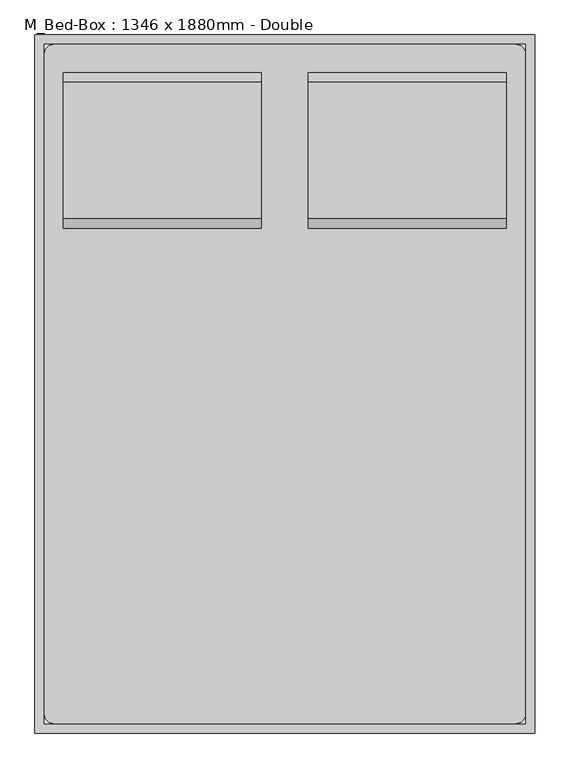
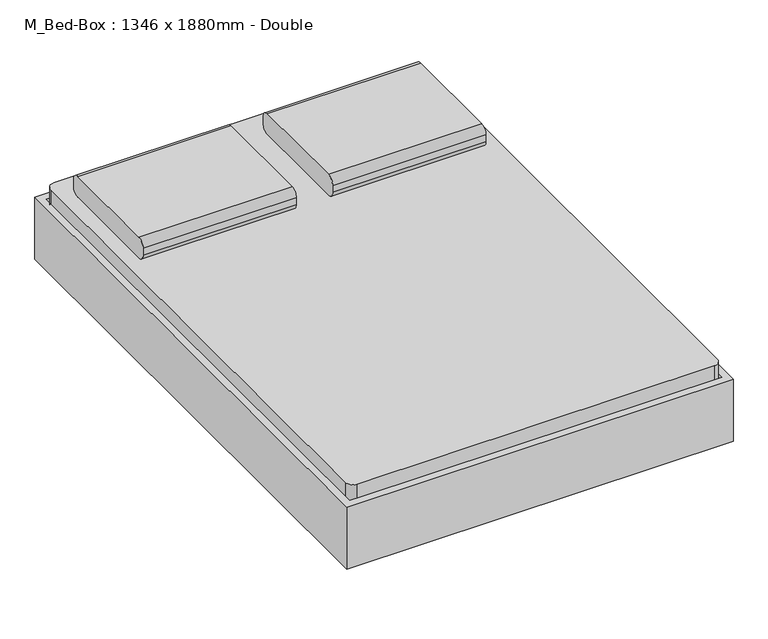
"""IFC4 building model written with IfcOpenShell, lengths in millimetres: furniture geometry, M_Bed-Box : 1346 x 1880mm - Double."""

import ifcopenshell
import ifcopenshell.guid

model = None  # the IFC model being written
_history = None  # IfcOwnerHistory: only IFC2X3 demands one
_inside = {}  # id of a spatial element -> (the spatial element, [elements in it])
_under = {}  # id of a project, library or spatial element -> (it, [spatial elements below it])
_declared = {}  # id of a project -> (the project, [libraries it declares])
_typed = {}  # id of a type object -> (the type object, [elements of that type])
_made_of = {}  # id of a material, layer set ... -> (it, [elements and type objects made of it])


def new_model(schema):
    """Start an empty IFC model of exactly this schema.

    Asked for "IFC4X3", IfcOpenShell would pick the latest addendum, in which some entities
    have other attributes; the version numbers below select the first issue.
    IFC2X3 requires an IfcOwnerHistory on every rooted entity: one is made here for all.
    """
    global model, _history
    if schema == "IFC4X3":
        model = ifcopenshell.file(schema_version=(4, 3, 0, 0))
    else:
        model = ifcopenshell.file(schema=schema)
    _inside.clear()
    _under.clear()
    _declared.clear()
    _typed.clear()
    _made_of.clear()
    _history = None
    if model.schema == "IFC2X3":
        org = make("IfcOrganization", Name="unknown")
        user = make(
            "IfcPersonAndOrganization",
            ThePerson=make("IfcPerson", FamilyName="unknown"),
            TheOrganization=org,
        )
        app = make(
            "IfcApplication",
            ApplicationDeveloper=org,
            Version="unknown",
            ApplicationFullName="unknown",
            ApplicationIdentifier="unknown",
        )
        _history = make(
            "IfcOwnerHistory",
            OwningUser=user,
            OwningApplication=app,
            ChangeAction="ADDED",
            CreationDate=0,
        )
    return model


def make(cls, **values):
    """One entity of the class cls with the attributes given. An attribute that is None is left unset."""
    return model.create_entity(
        cls, **{name: value for name, value in values.items() if value is not None}
    )


def rooted(cls, **values):
    """An entity with a GlobalId (a new one), such as an element, a storey or a relation."""
    return make(cls, GlobalId=ifcopenshell.guid.new(), OwnerHistory=_history, **values)


def si_unit(unit_type, name, prefix=None):
    """IfcSIUnit, for example si_unit("LENGTHUNIT", "METRE", prefix="MILLI")."""
    return make("IfcSIUnit", UnitType=unit_type, Prefix=prefix, Name=name)


def assignment(units):
    """IfcUnitAssignment: the units of a project."""
    return None if units is None else make("IfcUnitAssignment", Units=units)


def point(xyz):
    """IfcCartesianPoint."""
    return None if xyz is None else make("IfcCartesianPoint", Coordinates=xyz)


def direction(xyz):
    """IfcDirection."""
    return None if xyz is None else make("IfcDirection", DirectionRatios=xyz)


def frame(location, z_axis=None, x_axis=None):
    """IfcAxis2Placement3D, a coordinate frame: its origin and axes. An axis left out is left unset."""
    return make(
        "IfcAxis2Placement3D",
        Location=point(location),
        Axis=direction(z_axis),
        RefDirection=direction(x_axis),
    )


def frame_2d(location, x_axis=None):
    """IfcAxis2Placement2D, a coordinate frame in the plane: its origin and x axis."""
    return make(
        "IfcAxis2Placement2D", Location=point(location), RefDirection=direction(x_axis)
    )


def origin():
    """The frame at (0, 0, 0) with its axes left unset."""
    return frame((0.0, 0.0, 0.0))


def place(relative_to, where):
    """IfcLocalPlacement: puts the frame where relative to a parent placement (None: the world)."""
    return make(
        "IfcLocalPlacement", PlacementRelTo=relative_to, RelativePlacement=where
    )


def context(
    kind, dimensions, precision=None, world=None, true_north=None, identifier=None
):
    """IfcGeometricRepresentationContext, for example the 3D "Model" context."""
    return make(
        "IfcGeometricRepresentationContext",
        ContextIdentifier=identifier,
        ContextType=kind,
        CoordinateSpaceDimension=dimensions,
        Precision=precision,
        WorldCoordinateSystem=world,
        TrueNorth=true_north,
    )


def project(units=None, contexts=None):
    """IfcProject with its units and contexts."""
    return rooted(
        "IfcProject",
        Name="project",
        RepresentationContexts=contexts,
        UnitsInContext=assignment(units),
    )


def spatial(cls, under=None, at=None, **own):
    """A site, building, storey or space (cls), placed at a placement, below another one or the project."""
    s = rooted(cls, ObjectPlacement=at, **own)
    if under is not None:
        _under.setdefault(under.id(), (under, []))[1].append(s)
    return s


def polyline(points):
    """IfcPolyline through the points."""
    return make("IfcPolyline", Points=[point(p) for p in points])


def circle_curve(where, radius):
    """IfcCircle in the frame where."""
    return make("IfcCircle", Position=where, Radius=radius)


def trimmed(basis, trim1, trim2, sense, master):
    """IfcTrimmedCurve: the piece of a basis curve between two trims."""
    return make(
        "IfcTrimmedCurve",
        BasisCurve=basis,
        Trim1=trim1,
        Trim2=trim2,
        SenseAgreement=sense,
        MasterRepresentation=master,
    )


def segment(curve, same_sense, transition):
    """IfcCompositeCurveSegment."""
    return make(
        "IfcCompositeCurveSegment",
        Transition=transition,
        SameSense=same_sense,
        ParentCurve=curve,
    )


def composite_curve(segments, self_intersect=None):
    """IfcCompositeCurve: segments joined end to end."""
    return make("IfcCompositeCurve", Segments=segments, SelfIntersect=self_intersect)


def outline(outer, holes=None, kind="AREA"):
    """IfcArbitraryClosedProfileDef: a profile drawn as a closed curve; with holes, ...WithVoids."""
    if holes is None:
        return make("IfcArbitraryClosedProfileDef", ProfileType=kind, OuterCurve=outer)
    return make(
        "IfcArbitraryProfileDefWithVoids",
        ProfileType=kind,
        OuterCurve=outer,
        InnerCurves=holes,
    )


def extrude(swept, where, along, depth):
    """IfcExtrudedAreaSolid: the profile swept, set in the frame where, extruded along a direction by depth."""
    return make(
        "IfcExtrudedAreaSolid",
        SweptArea=swept,
        Position=where,
        ExtrudedDirection=direction(along),
        Depth=depth,
    )


def shape(context_of_items, identifier, shape_type, items):
    """IfcShapeRepresentation: the items that make up one representation, for example the "Body"."""
    return make(
        "IfcShapeRepresentation",
        ContextOfItems=context_of_items,
        RepresentationIdentifier=identifier,
        RepresentationType=shape_type,
        Items=items,
    )


def source(mapping_origin, context_of_items, identifier, shape_type, items):
    """IfcRepresentationMap: a shape defined once, which mapped items show again and again."""
    return make(
        "IfcRepresentationMap",
        MappingOrigin=mapping_origin,
        MappedRepresentation=shape(context_of_items, identifier, shape_type, items),
    )


def transform(
    local_origin,
    x_axis=None,
    y_axis=None,
    z_axis=None,
    scale=None,
    scale2=None,
    scale3=None,
    uniform=True,
):
    """IfcCartesianTransformationOperator3D, or its non-uniform kind. x_axis, y_axis, z_axis: its Axis1, 2, 3."""
    if uniform:
        return make(
            "IfcCartesianTransformationOperator3D",
            Axis1=direction(x_axis),
            Axis2=direction(y_axis),
            LocalOrigin=point(local_origin),
            Scale=scale,
            Axis3=direction(z_axis),
        )
    return make(
        "IfcCartesianTransformationOperator3DnonUniform",
        Axis1=direction(x_axis),
        Axis2=direction(y_axis),
        LocalOrigin=point(local_origin),
        Scale=scale,
        Axis3=direction(z_axis),
        Scale2=scale2,
        Scale3=scale3,
    )


def mapped(mapping_source, mapping_target):
    """IfcMappedItem: shows the shape of a source again, moved by a transform."""
    return make(
        "IfcMappedItem", MappingSource=mapping_source, MappingTarget=mapping_target
    )


def made_of(thing, what):
    """Note that an element or type object is made of a material, layer set ...; save() writes the relation."""
    if what is not None:
        _made_of.setdefault(what.id(), (what, []))[1].append(thing)
    return thing


def element(
    cls,
    number,
    at=None,
    inside=None,
    cuts=None,
    type_object=None,
    material=None,
    context=None,
    identifier="Body",
    shape_type=None,
    held_by="IfcProductDefinitionShape",
    body=None,
    shapes=None,
    **own,
):
    """One element of the class cls, such as IfcWall. Its Tag is "e" and its number.

    at: its placement. inside: the storey or other place that contains it. cuts: it is an
    opening in that element (IfcRelVoidsElement). A single representation is given by context,
    identifier, shape_type and body (its items); several are given by shapes. held_by: the class
    of the entity that holds the representations. save() writes the other relations.
    """
    e = rooted(cls, Tag="e%d" % number, ObjectPlacement=at, **own)
    if body is not None:
        shapes = [shape(context, identifier, shape_type, body)]
    if shapes is not None:
        e.Representation = make(held_by, Representations=shapes)
    if inside is not None:
        _inside.setdefault(inside.id(), (inside, []))[1].append(e)
    if cuts is not None:
        rooted(
            "IfcRelVoidsElement", RelatingBuildingElement=cuts, RelatedOpeningElement=e
        )
    if type_object is not None:
        _typed.setdefault(type_object.id(), (type_object, []))[1].append(e)
    return made_of(e, material)


def aggregate(whole, parts):
    """IfcRelAggregates: a whole, such as a stair, and the parts it consists of."""
    return rooted("IfcRelAggregates", RelatingObject=whole, RelatedObjects=parts)


def save(model, path):
    """Write the relations noted so far, then the file.

    IfcRelAggregates (storeys below a building ...), IfcRelContainedInSpatialStructure (elements
    in a storey), IfcRelDefinesByType, IfcRelAssociatesMaterial and IfcRelDeclares: one each for
    every whole, place, type object, material and project.
    """
    for whole, parts in _under.values():
        aggregate(whole, parts)
    for where, things in _inside.values():
        rooted(
            "IfcRelContainedInSpatialStructure",
            RelatedElements=things,
            RelatingStructure=where,
        )
    for kind, things in _typed.values():
        rooted("IfcRelDefinesByType", RelatedObjects=things, RelatingType=kind)
    for what, things in _made_of.values():
        rooted("IfcRelAssociatesMaterial", RelatedObjects=things, RelatingMaterial=what)
    for by, libraries in _declared.values():
        rooted("IfcRelDeclares", RelatingContext=by, RelatedDefinitions=libraries)
    model.write(path)


def plane_surface(at):
    """IfcPlane: the flat surface through the origin of the frame at, square to its z axis."""
    return make("IfcPlane", Position=at)


def cylinder_surface(at, radius):
    """IfcCylindricalSurface: all points at the distance radius from the z axis of the frame at."""
    return make("IfcCylindricalSurface", Position=at, Radius=radius)


def revolved_surface(curve, axis_point, axis_direction):
    """IfcSurfaceOfRevolution: the curve turned about the line through axis_point along axis_direction."""
    return make(
        "IfcSurfaceOfRevolution",
        SweptCurve=make("IfcArbitraryOpenProfileDef", ProfileType="CURVE", Curve=curve),
        AxisPosition=make("IfcAxis1Placement", Location=point(axis_point), Axis=direction(axis_direction)),
    )


def advanced_brep(points, edges, surfaces, faces):
    """IfcAdvancedBrep: a solid bounded by faces that lie on surfaces and meet in shared edges.

    An edge is (start, end): straight between two places in points (the first is 0);
    or (start, end, curve); or (start, end, curve, False) where it runs against its curve.
    A face is (place in surfaces, loops), or (place, loops, False) where it looks against
    its surface's normal. A loop lists edges by number (the first is 1), with a minus sign
    where the edge is run from its end to its start. The first loop is the outer one.
    """
    corners = [point(p) for p in points]
    vertices = [make("IfcVertexPoint", VertexGeometry=c) for c in corners]
    made = []
    for start, end, *more in edges:
        made.append(
            make(
                "IfcEdgeCurve",
                EdgeStart=vertices[start],
                EdgeEnd=vertices[end],
                EdgeGeometry=more[0] if more else make("IfcPolyline", Points=[corners[start], corners[end]]),
                SameSense=more[1] if len(more) > 1 else True,
            )
        )
    hull = []
    for where, loops, *sense in faces:
        bounds = []
        for j, loop in enumerate(loops):
            ring = [make("IfcOrientedEdge", EdgeElement=made[abs(k) - 1], Orientation=k > 0) for k in loop]
            bounds.append(
                make(
                    "IfcFaceOuterBound" if j == 0 else "IfcFaceBound",
                    Bound=make("IfcEdgeLoop", EdgeList=ring),
                    Orientation=True,
                )
            )
        hull.append(make("IfcAdvancedFace", Bounds=bounds, FaceSurface=surfaces[where], SameSense=sense[0] if sense else True))
    return make("IfcAdvancedBrep", Outer=make("IfcClosedShell", CfsFaces=hull))


def m_bed_box_1346_x_1880mm_double_b32eb57e(model_context):
    return source(origin(), model_context, "Body", "SolidModel", [
        extrude(outline(composite_curve([segment(polyline([(578.5704918, 406.4), (210.2704918, 406.4)]), True, "CONTINUOUS"), segment(trimmed(circle_curve(frame_2d((210.2704918, 431.8)), 25.4), [point((210.2704918, 406.4))], [point((184.8704918, 431.8))], False, "CARTESIAN"), True, "CONTINUOUS"), segment(polyline([(184.8704918, 431.8), (184.8704918, 457.2)]), True, "CONTINUOUS"), segment(trimmed(circle_curve(frame_2d((210.2704918, 457.2)), 25.4), [point((184.8704918, 457.2))], [point((210.2704918, 482.6))], False, "CARTESIAN"), True, "CONTINUOUS"), segment(polyline([(210.2704918, 482.6), (578.5704918, 482.6)]), True, "CONTINUOUS"), segment(trimmed(circle_curve(frame_2d((578.5704918, 457.2)), 25.4), [point((578.5704918, 482.6))], [point((603.9704918, 457.2))], False, "CARTESIAN"), True, "CONTINUOUS"), segment(polyline([(603.9704918, 457.2), (603.9704918, 431.8)]), True, "CONTINUOUS"), segment(trimmed(circle_curve(frame_2d((578.5704918, 431.8)), 25.4), [point((603.9704918, 431.8))], [point((578.5704918, 406.4))], False, "CARTESIAN"), True, "CONTINUOUS")], self_intersect=False)), frame((402.652459, 0.0, 0.0), z_axis=(1.0, 0.0, 0.0), x_axis=(0.0, 1.0, 0.0)), (0.0, 0.0, 1.0), 533.3),
        extrude(outline(composite_curve([segment(polyline([(578.5704918, 406.4), (210.2704918, 406.4)]), True, "CONTINUOUS"), segment(trimmed(circle_curve(frame_2d((210.2704918, 431.8)), 25.4), [point((210.2704918, 406.4))], [point((184.8704918, 431.8))], False, "CARTESIAN"), True, "CONTINUOUS"), segment(polyline([(184.8704918, 431.8), (184.8704918, 457.2)]), True, "CONTINUOUS"), segment(trimmed(circle_curve(frame_2d((210.2704918, 457.2)), 25.4), [point((184.8704918, 457.2))], [point((210.2704918, 482.6))], False, "CARTESIAN"), True, "CONTINUOUS"), segment(polyline([(210.2704918, 482.6), (578.5704918, 482.6)]), True, "CONTINUOUS"), segment(trimmed(circle_curve(frame_2d((578.5704918, 457.2)), 25.4), [point((578.5704918, 482.6))], [point((603.9704918, 457.2))], False, "CARTESIAN"), True, "CONTINUOUS"), segment(polyline([(603.9704918, 457.2), (603.9704918, 431.8)]), True, "CONTINUOUS"), segment(trimmed(circle_curve(frame_2d((578.5704918, 431.8)), 25.4), [point((603.9704918, 431.8))], [point((578.5704918, 406.4))], False, "CARTESIAN"), True, "CONTINUOUS")], self_intersect=False)), frame((-257.647541, 0.0, 0.0), z_axis=(1.0, 0.0, 0.0), x_axis=(0.0, 1.0, 0.0)), (0.0, 0.0, 1.0), 533.3),
        advanced_brep(
        [(-308.1231784, 451.5704918, 177.8), (-308.1231784, 375.3704918, 177.8), (-308.1231784, 375.3704918, 196.85), (-308.1231784, 451.5704918, 196.85), (-257.3231784, 451.5704918, 177.8), (-257.3231784, 375.3704918, 177.8), (-245.1869899, 375.3704918, 196.85), (-245.1869899, 451.5704918, 196.85), (-181.2523099, 451.5704918, 14.6654962), (-181.2523099, 375.3704918, 14.6654962), (-163.9871466, 375.3704918, 22.716374), (-163.9871466, 451.5704918, 22.716374), (-158.2320921, 375.3704918, 0.0), (-158.2320921, 451.5704918, 0.0), (-158.2320921, 375.3704918, 19.05), (-158.2320921, 451.5704918, 19.05), (-79.6195862, 451.5704918, 0.0), (-79.6195862, 375.3704918, 0.0), (-79.6195862, 375.3704918, 19.05), (-79.6195862, 451.5704918, 19.05), (-66.9195862, 375.3704918, 3.4029547), (-66.9195862, 451.5704918, 3.4029547), (-76.4445862, 375.3704918, 19.9007387), (-76.4445862, 451.5704918, 19.9007387), (-6.822541, 451.5704918, 38.1), (-6.822541, 375.3704918, 38.1), (-11.9269731, 375.3704918, 57.15), (-11.9269731, 451.5704918, 57.15), (685.4518216, 451.5704918, 38.1), (685.4518216, 375.3704918, 38.1), (690.5562537, 375.3704918, 57.15), (690.5562537, 451.5704918, 57.15), (745.5488669, 451.5704918, 3.4029547), (745.5488669, 375.3704918, 3.4029547), (755.0738669, 375.3704918, 19.9007387), (755.0738669, 451.5704918, 19.9007387), (758.2488669, 375.3704918, 0.0), (758.2488669, 451.5704918, 0.0), (758.2488669, 375.3704918, 19.05), (758.2488669, 451.5704918, 19.05), (836.8613728, 451.5704918, 0.0), (836.8613728, 375.3704918, 0.0), (836.8613728, 375.3704918, 19.05), (836.8613728, 451.5704918, 19.05), (859.8815906, 375.3704918, 14.6654962), (859.8815906, 451.5704918, 14.6654962), (842.6164272, 375.3704918, 22.716374), (842.6164272, 451.5704918, 22.716374), (935.952459, 451.5704918, 177.8), (935.952459, 375.3704918, 177.8), (923.8162705, 375.3704918, 196.85), (923.8162705, 451.5704918, 196.85), (986.752459, 451.5704918, 177.8), (986.752459, 451.5704918, 196.85), (986.752459, 375.3704918, 196.85), (986.752459, 375.3704918, 177.8)],
        [
            (0, 1),
            (1, 2),
            (2, 3),
            (3, 0),
            (0, 4),
            (4, 5),
            (5, 1),
            (5, 6),
            (6, 2),
            (6, 7),
            (7, 3),
            (7, 4),
            (4, 8),
            (8, 9),
            (9, 5),
            (9, 10),
            (10, 6),
            (10, 11),
            (11, 7),
            (11, 8),
            (12, 9, circle_curve(frame((-158.2320921, 375.3704918, 25.4), z_axis=(0.0, 1.0, 0.0), x_axis=(-0.906307787036649, 0.0, -0.4226182617407015)), 25.4)),
            (8, 13, circle_curve(frame((-158.2320921, 451.5704918, 25.4), z_axis=(0.0, -1.0, 0.0), x_axis=(-0.906307787036649, 0.0, -0.4226182617407015)), 25.4)),
            (13, 12),
            (14, 10, circle_curve(frame((-158.2320921, 375.3704918, 25.4), z_axis=(0.0, 1.0, 0.0), x_axis=(-0.906307787036649, 0.0, -0.4226182617407015)), 6.35)),
            (12, 14),
            (15, 11, circle_curve(frame((-158.2320921, 451.5704918, 25.4), z_axis=(0.0, 1.0, 0.0), x_axis=(-0.906307787036649, 0.0, -0.4226182617407015)), 6.35)),
            (14, 15),
            (15, 13),
            (13, 16),
            (16, 17),
            (17, 12),
            (17, 18),
            (18, 14),
            (18, 19),
            (19, 15),
            (19, 16),
            (20, 17, circle_curve(frame((-79.6195862, 375.3704918, 25.4), z_axis=(0.0, 1.0, 0.0), x_axis=(0.0, 0.0, -1.0)), 25.4)),
            (16, 21, circle_curve(frame((-79.6195862, 451.5704918, 25.4), z_axis=(0.0, -1.0, 0.0), x_axis=(0.0, 0.0, -1.0)), 25.4)),
            (21, 20),
            (22, 18, circle_curve(frame((-79.6195862, 375.3704918, 25.4), z_axis=(0.0, 1.0, 0.0), x_axis=(0.0, 0.0, -1.0)), 6.35)),
            (20, 22),
            (23, 19, circle_curve(frame((-79.6195862, 451.5704918, 25.4), z_axis=(0.0, 1.0, 0.0), x_axis=(0.0, 0.0, -1.0)), 6.35)),
            (22, 23),
            (23, 21),
            (21, 24),
            (24, 25),
            (25, 20),
            (25, 26),
            (26, 22),
            (26, 27),
            (27, 23),
            (27, 24),
            (24, 28),
            (28, 29),
            (29, 25),
            (29, 30),
            (30, 26),
            (30, 31),
            (31, 27),
            (31, 28),
            (28, 32),
            (32, 33),
            (33, 29),
            (33, 34),
            (34, 30),
            (34, 35),
            (35, 31),
            (35, 32),
            (36, 33, circle_curve(frame((758.2488669, 375.3704918, 25.4), z_axis=(0.0, 1.0, 0.0), x_axis=(-0.5000000000000463, 0.0, -0.8660254037844118)), 25.4)),
            (32, 37, circle_curve(frame((758.2488669, 451.5704918, 25.4), z_axis=(0.0, -1.0, 0.0), x_axis=(-0.5000000000000463, 0.0, -0.8660254037844118)), 25.4)),
            (37, 36),
            (38, 34, circle_curve(frame((758.2488669, 375.3704918, 25.4), z_axis=(0.0, 1.0, 0.0), x_axis=(-0.5000000000000463, 0.0, -0.8660254037844118)), 6.35)),
            (36, 38),
            (39, 35, circle_curve(frame((758.2488669, 451.5704918, 25.4), z_axis=(0.0, 1.0, 0.0), x_axis=(-0.5000000000000463, 0.0, -0.8660254037844118)), 6.35)),
            (38, 39),
            (39, 37),
            (37, 40),
            (40, 41),
            (41, 36),
            (41, 42),
            (42, 38),
            (42, 43),
            (43, 39),
            (43, 40),
            (44, 41, circle_curve(frame((836.8613728, 375.3704918, 25.4), z_axis=(0.0, 1.0, 0.0), x_axis=(0.0, 0.0, -1.0)), 25.4)),
            (40, 45, circle_curve(frame((836.8613728, 451.5704918, 25.4), z_axis=(0.0, -1.0, 0.0), x_axis=(0.0, 0.0, -1.0)), 25.4)),
            (45, 44),
            (46, 42, circle_curve(frame((836.8613728, 375.3704918, 25.4), z_axis=(0.0, 1.0, 0.0), x_axis=(0.0, 0.0, -1.0)), 6.35)),
            (44, 46),
            (47, 43, circle_curve(frame((836.8613728, 451.5704918, 25.4), z_axis=(0.0, 1.0, 0.0), x_axis=(0.0, 0.0, -1.0)), 6.35)),
            (46, 47),
            (47, 45),
            (45, 48),
            (48, 49),
            (49, 44),
            (49, 50),
            (50, 46),
            (50, 51),
            (51, 47),
            (51, 48),
            (52, 53),
            (53, 54),
            (54, 55),
            (55, 52),
            (48, 52),
            (55, 49),
            (54, 50),
            (53, 51),
        ],
        [
            plane_surface(frame((-308.1231784, 705.5704918, -152.9490627), z_axis=(-1.0, 0.0, 0.0), x_axis=(0.0, 1.0, 0.0))),
            plane_surface(frame((-308.1231784, 451.5704918, 177.8), z_axis=(0.0, 0.0, -1.0), x_axis=(1.0, 0.0, 0.0))),
            plane_surface(frame((-308.1231784, 375.3704918, 177.8), z_axis=(0.0, -1.0, 0.0), x_axis=(1.0, 0.0, 0.0))),
            plane_surface(frame((-308.1231784, 375.3704918, 196.85), z_axis=(0.0, 0.0, 1.0), x_axis=(1.0, 0.0, 0.0))),
            plane_surface(frame((-308.1231784, 451.5704918, 196.85), z_axis=(0.0, 1.0, 0.0), x_axis=(1.0, 0.0, 0.0))),
            plane_surface(frame((-257.3231784, 451.5704918, 177.8), z_axis=(-0.9063077870366486, 0.0, -0.4226182617407026), x_axis=(0.4226182617407026, 0.0, -0.9063077870366486))),
            plane_surface(frame((-257.3231784, 375.3704918, 177.8), z_axis=(0.0, -1.0000000000000002, 0.0), x_axis=(0.4226182617407026, 0.0, -0.9063077870366486))),
            plane_surface(frame((-245.1869899, 375.3704918, 196.85), z_axis=(0.9063077870366487, 0.0, 0.4226182617407023), x_axis=(0.4226182617407023, 0.0, -0.9063077870366487))),
            plane_surface(frame((-245.1869899, 451.5704918, 196.85), z_axis=(0.0, 1.0, 0.0), x_axis=(0.4226182617407027, 0.0, -0.9063077870366485))),
            cylinder_surface(frame((-158.2320921, 705.5704918, 25.4), z_axis=(0.0, -1.0, 0.0), x_axis=(-0.906307787036649, 0.0, -0.4226182617407015)), 25.4),
            plane_surface(frame((-158.2320921, 375.3704918, 25.4), z_axis=(0.0, -1.0, 0.0), x_axis=(-0.906307787036649, 0.0, -0.4226182617407015))),
            revolved_surface(polyline([(-163.9871465476827, 375.3704918, 22.716374037946544), (-163.9871465476827, 451.5704918, 22.716374037946544)]), (-158.2320921, 705.5704918, 25.4), (0.0, -1.0, 0.0)),
            plane_surface(frame((-158.2320921, 451.5704918, 25.4), z_axis=(0.0, 1.0, 0.0), x_axis=(-0.906307787036649, 0.0, -0.4226182617407015))),
            plane_surface(frame((-158.2320921, 451.5704918, 0.0), z_axis=(0.0, 0.0, -1.0), x_axis=(1.0, 0.0, 0.0))),
            plane_surface(frame((-158.2320921, 375.3704918, 0.0), z_axis=(0.0, -1.0, 0.0), x_axis=(1.0, 0.0, 0.0))),
            plane_surface(frame((-158.2320921, 375.3704918, 19.05), z_axis=(0.0, 0.0, 1.0), x_axis=(1.0, 0.0, 0.0))),
            plane_surface(frame((-158.2320921, 451.5704918, 19.05), z_axis=(0.0, 1.0, 0.0), x_axis=(1.0, 0.0, 0.0))),
            cylinder_surface(frame((-79.6195862, 705.5704918, 25.4), z_axis=(0.0, -1.0, 0.0), x_axis=(0.0, 0.0, -1.0)), 25.4),
            plane_surface(frame((-79.6195862, 375.3704918, 25.4), z_axis=(0.0, -1.0, 0.0), x_axis=(0.0, 0.0, -1.0))),
            revolved_surface(polyline([(-79.6195862, 375.3704918, 19.049999999999997), (-79.6195862, 451.5704918, 19.049999999999997)]), (-79.6195862, 705.5704918, 25.4), (0.0, -1.0, 0.0)),
            plane_surface(frame((-79.6195862, 451.5704918, 25.4), z_axis=(0.0, 1.0, 0.0), x_axis=(0.0, 0.0, -1.0))),
            plane_surface(frame((-66.9195862, 451.5704918, 3.4029547), z_axis=(0.4999999999998744, 0.0, -0.8660254037845112), x_axis=(0.8660254037845112, 0.0, 0.4999999999998744))),
            plane_surface(frame((-66.9195862, 375.3704918, 3.4029547), z_axis=(0.0, -1.0000000000000002, 0.0), x_axis=(0.8660254037845112, 0.0, 0.4999999999998745))),
            plane_surface(frame((-76.4445862, 375.3704918, 19.9007387), z_axis=(-0.4999999999998741, 0.0, 0.8660254037845113), x_axis=(0.8660254037845113, 0.0, 0.4999999999998741))),
            plane_surface(frame((-76.4445862, 451.5704918, 19.9007387), z_axis=(0.0, 1.0, 0.0), x_axis=(0.866025403784511, 0.0, 0.49999999999987477))),
            plane_surface(frame((-6.822541, 451.5704918, 38.1), z_axis=(0.0, 0.0, -1.0), x_axis=(1.0, 0.0, 0.0))),
            plane_surface(frame((-6.822541, 375.3704918, 38.1), z_axis=(0.0, -1.0, 0.0), x_axis=(1.0, 0.0, 0.0))),
            plane_surface(frame((-11.9269731, 375.3704918, 57.15), z_axis=(0.0, 0.0, 1.0), x_axis=(1.0, 0.0, 0.0))),
            plane_surface(frame((-11.9269731, 451.5704918, 57.15), z_axis=(0.0, 1.0, 0.0), x_axis=(1.0, 0.0, 0.0))),
            plane_surface(frame((685.4518216, 451.5704918, 38.1), z_axis=(-0.5000000000000494, 0.0, -0.8660254037844102), x_axis=(0.8660254037844102, 0.0, -0.5000000000000494))),
            plane_surface(frame((685.4518216, 375.3704918, 38.1), z_axis=(0.0, -1.0, 0.0), x_axis=(0.8660254037844112, 0.0, -0.5000000000000476))),
            plane_surface(frame((690.5562537, 375.3704918, 57.15), z_axis=(0.5000000000000488, 0.0, 0.8660254037844105), x_axis=(0.8660254037844105, 0.0, -0.5000000000000488))),
            plane_surface(frame((690.5562537, 451.5704918, 57.15), z_axis=(0.0, 1.0, 0.0), x_axis=(0.8660254037844106, 0.0, -0.5000000000000485))),
            cylinder_surface(frame((758.2488669, 705.5704918, 25.4), z_axis=(0.0, -1.0, 0.0), x_axis=(-0.5000000000000463, 0.0, -0.8660254037844118)), 25.4),
            plane_surface(frame((758.2488669, 375.3704918, 25.4), z_axis=(0.0, -1.0000000000000002, 0.0), x_axis=(-0.5000000000000464, 0.0, -0.866025403784412))),
            revolved_surface(polyline([(755.0738668999998, 375.3704918, 19.90073868596898), (755.0738668999998, 451.5704918, 19.90073868596898)]), (758.2488669, 705.5704918, 25.4), (0.0, -1.0, 0.0)),
            plane_surface(frame((758.2488669, 451.5704918, 25.4), z_axis=(0.0, 1.0000000000000002, 0.0), x_axis=(-0.5000000000000464, 0.0, -0.866025403784412))),
            plane_surface(frame((758.2488669, 451.5704918, 0.0), z_axis=(0.0, 0.0, -1.0), x_axis=(1.0, 0.0, 0.0))),
            plane_surface(frame((758.2488669, 375.3704918, 0.0), z_axis=(0.0, -1.0, 0.0), x_axis=(1.0, 0.0, 0.0))),
            plane_surface(frame((758.2488669, 375.3704918, 19.05), z_axis=(0.0, 0.0, 1.0), x_axis=(1.0, 0.0, 0.0))),
            plane_surface(frame((758.2488669, 451.5704918, 19.05), z_axis=(0.0, 1.0, 0.0), x_axis=(1.0, 0.0, 0.0))),
            cylinder_surface(frame((836.8613728, 705.5704918, 25.4), z_axis=(0.0, -1.0, 0.0), x_axis=(0.0, 0.0, -1.0)), 25.4),
            plane_surface(frame((836.8613728, 375.3704918, 25.4), z_axis=(0.0, -1.0, 0.0), x_axis=(0.0, 0.0, -1.0))),
            revolved_surface(polyline([(836.8613728, 375.3704918, 19.049999999999997), (836.8613728, 451.5704918, 19.049999999999997)]), (836.8613728, 705.5704918, 25.4), (0.0, -1.0, 0.0)),
            plane_surface(frame((836.8613728, 451.5704918, 25.4), z_axis=(0.0, 1.0, 0.0), x_axis=(0.0, 0.0, -1.0))),
            plane_surface(frame((859.8815906, 451.5704918, 14.6654962), z_axis=(0.90630778703668, 0.0, -0.422618261740635), x_axis=(0.422618261740635, 0.0, 0.90630778703668))),
            plane_surface(frame((859.8815906, 375.3704918, 14.6654962), z_axis=(0.0, -1.0000000000000002, 0.0), x_axis=(0.4226182617406349, 0.0, 0.9063077870366801))),
            plane_surface(frame((842.6164272, 375.3704918, 22.716374), z_axis=(-0.9063077870366805, 0.0, 0.4226182617406341), x_axis=(0.4226182617406341, 0.0, 0.9063077870366805))),
            plane_surface(frame((842.6164272, 451.5704918, 22.716374), z_axis=(0.0, 1.0, 0.0), x_axis=(0.42261826174063455, 0.0, 0.9063077870366802))),
            plane_surface(frame((986.752459, 705.5704918, -152.9490627), z_axis=(1.0, 0.0, 0.0), x_axis=(0.0, 1.0, 0.0))),
            plane_surface(frame((935.952459, 451.5704918, 177.8), z_axis=(0.0, 0.0, -1.0), x_axis=(1.0, 0.0, 0.0))),
            plane_surface(frame((935.952459, 375.3704918, 177.8), z_axis=(0.0, -1.0, 0.0), x_axis=(1.0, 0.0, 0.0))),
            plane_surface(frame((923.8162705, 375.3704918, 196.85), z_axis=(0.0, 0.0, 1.0), x_axis=(1.0, 0.0, 0.0))),
            plane_surface(frame((923.8162705, 451.5704918, 196.85), z_axis=(0.0, 1.0, 0.0), x_axis=(1.0, 0.0, 0.0))),
        ],
        [
            (0, [[1, 2, 3, 4]]),
            (1, [[-1, 5, 6, 7]]),
            (2, [[-2, -7, 8, 9]]),
            (3, [[-3, -9, 10, 11]]),
            (4, [[-4, -11, 12, -5]]),
            (5, [[-6, 13, 14, 15]]),
            (6, [[-8, -15, 16, 17]]),
            (7, [[-10, -17, 18, 19]]),
            (8, [[-12, -19, 20, -13]]),
            (9, [[21, -14, 22, 23]]),
            (10, [[24, -16, -21, 25]]),
            (11, [[26, -18, -24, 27]]),
            (12, [[-22, -20, -26, 28]]),
            (13, [[-23, 29, 30, 31]]),
            (14, [[-25, -31, 32, 33]]),
            (15, [[-27, -33, 34, 35]]),
            (16, [[-28, -35, 36, -29]]),
            (17, [[37, -30, 38, 39]]),
            (18, [[40, -32, -37, 41]]),
            (19, [[42, -34, -40, 43]]),
            (20, [[-38, -36, -42, 44]]),
            (21, [[-39, 45, 46, 47]]),
            (22, [[-41, -47, 48, 49]]),
            (23, [[-43, -49, 50, 51]]),
            (24, [[-44, -51, 52, -45]]),
            (25, [[-46, 53, 54, 55]]),
            (26, [[-48, -55, 56, 57]]),
            (27, [[-50, -57, 58, 59]]),
            (28, [[-52, -59, 60, -53]]),
            (29, [[-54, 61, 62, 63]]),
            (30, [[-56, -63, 64, 65]]),
            (31, [[-58, -65, 66, 67]]),
            (32, [[-60, -67, 68, -61]]),
            (33, [[69, -62, 70, 71]]),
            (34, [[72, -64, -69, 73]]),
            (35, [[74, -66, -72, 75]]),
            (36, [[-70, -68, -74, 76]]),
            (37, [[-71, 77, 78, 79]]),
            (38, [[-73, -79, 80, 81]]),
            (39, [[-75, -81, 82, 83]]),
            (40, [[-76, -83, 84, -77]]),
            (41, [[85, -78, 86, 87]]),
            (42, [[88, -80, -85, 89]]),
            (43, [[90, -82, -88, 91]]),
            (44, [[-86, -84, -90, 92]]),
            (45, [[-87, 93, 94, 95]]),
            (46, [[-89, -95, 96, 97]]),
            (47, [[-91, -97, 98, 99]]),
            (48, [[-92, -99, 100, -93]]),
            (49, [[101, 102, 103, 104]]),
            (50, [[-94, 105, -104, 106]]),
            (51, [[-96, -106, -103, 107]]),
            (52, [[-98, -107, -102, 108]]),
            (53, [[-100, -108, -101, -105]]),
        ],
    ),
        extrude(outline(composite_curve([segment(polyline([(-283.047541, 680.1704918), (961.352459, 680.1704918)]), True, "CONTINUOUS"), segment(trimmed(circle_curve(frame_2d((961.352459, 654.7704918)), 25.4), [point((961.352459, 680.1704918))], [point((986.752459, 654.7704918))], False, "CARTESIAN"), True, "CONTINUOUS"), segment(polyline([(986.752459, 654.7704918), (986.752459, -1123.6295082)]), True, "CONTINUOUS"), segment(trimmed(circle_curve(frame_2d((961.352459, -1123.6295082)), 25.4), [point((986.752459, -1123.6295082))], [point((961.352459, -1149.0295082))], False, "CARTESIAN"), True, "CONTINUOUS"), segment(polyline([(961.352459, -1149.0295082), (-283.047541, -1149.0295082)]), True, "CONTINUOUS"), segment(trimmed(circle_curve(frame_2d((-283.047541, -1123.6295082)), 25.4), [point((-283.047541, -1149.0295082))], [point((-308.447541, -1123.6295082))], False, "CARTESIAN"), True, "CONTINUOUS"), segment(polyline([(-308.447541, -1123.6295082), (-308.447541, 654.7704918)]), True, "CONTINUOUS"), segment(trimmed(circle_curve(frame_2d((-283.047541, 654.7704918)), 25.4), [point((-308.447541, 654.7704918))], [point((-283.047541, 680.1704918))], False, "CARTESIAN"), True, "CONTINUOUS")], self_intersect=False)), frame((0.0, 0.0, 203.2), z_axis=(0.0, 0.0, 1.0), x_axis=(1.0, 0.0, 0.0)), (0.0, 0.0, 1.0), 203.2),
        advanced_brep(
        [(-308.447541, -869.6295082, 196.85), (-308.447541, -869.6295082, 177.8), (-308.447541, -945.8295082, 177.8), (-308.447541, -945.8295082, 196.85), (-245.5113525, -869.6295082, 196.85), (-257.647541, -869.6295082, 177.8), (-257.647541, -945.8295082, 177.8), (-245.5113525, -945.8295082, 196.85), (-164.3115092, -869.6295082, 22.716374), (-181.5766725, -869.6295082, 14.6654962), (-181.5766725, -945.8295082, 14.6654962), (-164.3115092, -945.8295082, 22.716374), (-158.5564547, -869.6295082, 0.0), (-158.5564547, -869.6295082, 19.05), (-158.5564547, -945.8295082, 0.0), (-158.5564547, -945.8295082, 19.05), (-79.9439489, -869.6295082, 19.05), (-79.9439489, -869.6295082, 0.0), (-79.9439489, -945.8295082, 0.0), (-79.9439489, -945.8295082, 19.05), (-67.2439489, -869.6295082, 3.4029547), (-76.7689489, -869.6295082, 19.9007387), (-67.2439489, -945.8295082, 3.4029547), (-76.7689489, -945.8295082, 19.9007387), (-12.2513357, -869.6295082, 57.15), (-7.1469036, -869.6295082, 38.1), (-7.1469036, -945.8295082, 38.1), (-12.2513357, -945.8295082, 57.15), (690.5562537, -869.6295082, 57.15), (685.4518216, -869.6295082, 38.1), (685.4518216, -945.8295082, 38.1), (690.5562537, -945.8295082, 57.15), (755.0738669, -869.6295082, 19.9007387), (745.5488669, -869.6295082, 3.4029547), (745.5488669, -945.8295082, 3.4029547), (755.0738669, -945.8295082, 19.9007387), (758.2488669, -869.6295082, 0.0), (758.2488669, -869.6295082, 19.05), (758.2488669, -945.8295082, 0.0), (758.2488669, -945.8295082, 19.05), (836.8613728, -869.6295082, 19.05), (836.8613728, -869.6295082, 0.0), (836.8613728, -945.8295082, 0.0), (836.8613728, -945.8295082, 19.05), (859.8815906, -869.6295082, 14.6654962), (842.6164272, -869.6295082, 22.716374), (859.8815906, -945.8295082, 14.6654962), (842.6164272, -945.8295082, 22.716374), (923.8162705, -869.6295082, 196.85), (935.952459, -869.6295082, 177.8), (935.952459, -945.8295082, 177.8), (923.8162705, -945.8295082, 196.85), (986.752459, -869.6295082, 196.85), (986.752459, -945.8295082, 196.85), (986.752459, -945.8295082, 177.8), (986.752459, -869.6295082, 177.8)],
        [
            (0, 1),
            (1, 2),
            (2, 3),
            (3, 0),
            (0, 4),
            (4, 5),
            (5, 1),
            (5, 6),
            (6, 2),
            (6, 7),
            (7, 3),
            (7, 4),
            (4, 8),
            (8, 9),
            (9, 5),
            (9, 10),
            (10, 6),
            (10, 11),
            (11, 7),
            (11, 8),
            (12, 9, circle_curve(frame((-158.5564547, -869.6295082, 25.4), z_axis=(0.0, 1.0, 0.0), x_axis=(-0.9063077870366625, 0.0, -0.4226182617406725)), 25.4)),
            (8, 13, circle_curve(frame((-158.5564547, -869.6295082, 25.4), z_axis=(0.0, -1.0, 0.0), x_axis=(-0.9063077870366625, 0.0, -0.4226182617406725)), 6.35)),
            (13, 12),
            (14, 10, circle_curve(frame((-158.5564547, -945.8295082, 25.4), z_axis=(0.0, 1.0, 0.0), x_axis=(-0.9063077870366625, 0.0, -0.4226182617406725)), 25.4)),
            (12, 14),
            (15, 11, circle_curve(frame((-158.5564547, -945.8295082, 25.4), z_axis=(0.0, 1.0, 0.0), x_axis=(-0.9063077870366625, 0.0, -0.4226182617406725)), 6.35)),
            (14, 15),
            (15, 13),
            (13, 16),
            (16, 17),
            (17, 12),
            (17, 18),
            (18, 14),
            (18, 19),
            (19, 15),
            (19, 16),
            (20, 17, circle_curve(frame((-79.9439489, -869.6295082, 25.4), z_axis=(0.0, 1.0, 0.0), x_axis=(0.0, 0.0, -1.0)), 25.4)),
            (16, 21, circle_curve(frame((-79.9439489, -869.6295082, 25.4), z_axis=(0.0, -1.0, 0.0), x_axis=(0.0, 0.0, -1.0)), 6.35)),
            (21, 20),
            (22, 18, circle_curve(frame((-79.9439489, -945.8295082, 25.4), z_axis=(0.0, 1.0, 0.0), x_axis=(0.0, 0.0, -1.0)), 25.4)),
            (20, 22),
            (23, 19, circle_curve(frame((-79.9439489, -945.8295082, 25.4), z_axis=(0.0, 1.0, 0.0), x_axis=(0.0, 0.0, -1.0)), 6.35)),
            (22, 23),
            (23, 21),
            (21, 24),
            (24, 25),
            (25, 20),
            (25, 26),
            (26, 22),
            (26, 27),
            (27, 23),
            (27, 24),
            (24, 28),
            (28, 29),
            (29, 25),
            (29, 30),
            (30, 26),
            (30, 31),
            (31, 27),
            (31, 28),
            (28, 32),
            (32, 33),
            (33, 29),
            (33, 34),
            (34, 30),
            (34, 35),
            (35, 31),
            (35, 32),
            (36, 33, circle_curve(frame((758.2488669, -869.6295082, 25.4), z_axis=(0.0, 1.0, 0.0), x_axis=(-0.5000000000000528, 0.0, -0.8660254037844081)), 25.4)),
            (32, 37, circle_curve(frame((758.2488669, -869.6295082, 25.4), z_axis=(0.0, -1.0, 0.0), x_axis=(-0.5000000000000528, 0.0, -0.8660254037844081)), 6.35)),
            (37, 36),
            (38, 34, circle_curve(frame((758.2488669, -945.8295082, 25.4), z_axis=(0.0, 1.0, 0.0), x_axis=(-0.5000000000000528, 0.0, -0.8660254037844081)), 25.4)),
            (36, 38),
            (39, 35, circle_curve(frame((758.2488669, -945.8295082, 25.4), z_axis=(0.0, 1.0, 0.0), x_axis=(-0.5000000000000528, 0.0, -0.8660254037844081)), 6.35)),
            (38, 39),
            (39, 37),
            (37, 40),
            (40, 41),
            (41, 36),
            (41, 42),
            (42, 38),
            (42, 43),
            (43, 39),
            (43, 40),
            (44, 41, circle_curve(frame((836.8613728, -869.6295082, 25.4), z_axis=(0.0, 1.0, 0.0), x_axis=(0.0, 0.0, -1.0)), 25.4)),
            (40, 45, circle_curve(frame((836.8613728, -869.6295082, 25.4), z_axis=(0.0, -1.0, 0.0), x_axis=(0.0, 0.0, -1.0)), 6.35)),
            (45, 44),
            (46, 42, circle_curve(frame((836.8613728, -945.8295082, 25.4), z_axis=(0.0, 1.0, 0.0), x_axis=(0.0, 0.0, -1.0)), 25.4)),
            (44, 46),
            (47, 43, circle_curve(frame((836.8613728, -945.8295082, 25.4), z_axis=(0.0, 1.0, 0.0), x_axis=(0.0, 0.0, -1.0)), 6.35)),
            (46, 47),
            (47, 45),
            (45, 48),
            (48, 49),
            (49, 44),
            (49, 50),
            (50, 46),
            (50, 51),
            (51, 47),
            (51, 48),
            (52, 53),
            (53, 54),
            (54, 55),
            (55, 52),
            (48, 52),
            (55, 49),
            (54, 50),
            (53, 51),
        ],
        [
            plane_surface(frame((-308.447541, -1174.4295082, -127.5947323), z_axis=(-1.0, 0.0, 0.0), x_axis=(0.0, 1.0, 0.0))),
            plane_surface(frame((-308.447541, -869.6295082, 196.85), z_axis=(0.0, 1.0, 0.0), x_axis=(1.0, 0.0, 0.0))),
            plane_surface(frame((-308.447541, -869.6295082, 177.8), z_axis=(0.0, 0.0, -1.0), x_axis=(1.0, 0.0, 0.0))),
            plane_surface(frame((-308.447541, -945.8295082, 177.8), z_axis=(0.0, -1.0, 0.0), x_axis=(1.0, 0.0, 0.0))),
            plane_surface(frame((-308.447541, -945.8295082, 196.85), z_axis=(0.0, 0.0, 1.0), x_axis=(1.0, 0.0, 0.0))),
            plane_surface(frame((-245.5113525, -869.6295082, 196.85), z_axis=(0.0, 1.0, 0.0), x_axis=(0.4226182617406714, 0.0, -0.906307787036663))),
            plane_surface(frame((-257.647541, -869.6295082, 177.8), z_axis=(-0.9063077870366631, 0.0, -0.42261826174067146), x_axis=(0.42261826174067146, 0.0, -0.9063077870366631))),
            plane_surface(frame((-257.647541, -945.8295082, 177.8), z_axis=(0.0, -1.0000000000000002, 0.0), x_axis=(0.4226182617406716, 0.0, -0.906307787036663))),
            plane_surface(frame((-245.5113525, -945.8295082, 196.85), z_axis=(0.906307787036663, 0.0, 0.4226182617406716), x_axis=(0.4226182617406716, 0.0, -0.906307787036663))),
            plane_surface(frame((-158.5564547, -869.6295082, 25.4), z_axis=(0.0, 1.0, 0.0), x_axis=(-0.9063077870366625, 0.0, -0.4226182617406725))),
            cylinder_surface(frame((-158.5564547, -1174.4295082, 25.4), z_axis=(0.0, -1.0, 0.0), x_axis=(-0.9063077870366625, 0.0, -0.4226182617406725)), 25.4),
            plane_surface(frame((-158.5564547, -945.8295082, 25.4), z_axis=(0.0, -1.0, 0.0), x_axis=(-0.9063077870366625, 0.0, -0.4226182617406725))),
            revolved_surface(polyline([(-164.31150914768278, -945.8295082, 22.71637403794673), (-164.31150914768278, -869.6295082, 22.71637403794673)]), (-158.5564547, -1174.4295082, 25.4), (0.0, -1.0, 0.0)),
            plane_surface(frame((-158.5564547, -869.6295082, 19.05), z_axis=(0.0, 1.0, 0.0), x_axis=(1.0, 0.0, 0.0))),
            plane_surface(frame((-158.5564547, -869.6295082, 0.0), z_axis=(0.0, 0.0, -1.0), x_axis=(1.0, 0.0, 0.0))),
            plane_surface(frame((-158.5564547, -945.8295082, 0.0), z_axis=(0.0, -1.0, 0.0), x_axis=(1.0, 0.0, 0.0))),
            plane_surface(frame((-158.5564547, -945.8295082, 19.05), z_axis=(0.0, 0.0, 1.0), x_axis=(1.0, 0.0, 0.0))),
            plane_surface(frame((-79.9439489, -869.6295082, 25.4), z_axis=(0.0, 1.0, 0.0), x_axis=(0.0, 0.0, -1.0))),
            cylinder_surface(frame((-79.9439489, -1174.4295082, 25.4), z_axis=(0.0, -1.0, 0.0), x_axis=(0.0, 0.0, -1.0)), 25.4),
            plane_surface(frame((-79.9439489, -945.8295082, 25.4), z_axis=(0.0, -1.0, 0.0), x_axis=(0.0, 0.0, -1.0))),
            revolved_surface(polyline([(-79.9439489, -945.8295082, 19.049999999999997), (-79.9439489, -869.6295082, 19.049999999999997)]), (-79.9439489, -1174.4295082, 25.4), (0.0, -1.0, 0.0)),
            plane_surface(frame((-76.7689489, -869.6295082, 19.9007387), z_axis=(0.0, 1.0000000000000002, 0.0), x_axis=(0.8660254037844788, 0.0, 0.49999999999993067))),
            plane_surface(frame((-67.2439489, -869.6295082, 3.4029547), z_axis=(0.49999999999993067, 0.0, -0.8660254037844787), x_axis=(0.8660254037844787, 0.0, 0.49999999999993067))),
            plane_surface(frame((-67.2439489, -945.8295082, 3.4029547), z_axis=(0.0, -1.0, 0.0), x_axis=(0.8660254037844782, 0.0, 0.4999999999999315))),
            plane_surface(frame((-76.7689489, -945.8295082, 19.9007387), z_axis=(-0.49999999999993044, 0.0, 0.8660254037844789), x_axis=(0.8660254037844789, 0.0, 0.49999999999993044))),
            plane_surface(frame((-12.2513357, -869.6295082, 57.15), z_axis=(0.0, 1.0, 0.0), x_axis=(1.0, 0.0, 0.0))),
            plane_surface(frame((-7.1469036, -869.6295082, 38.1), z_axis=(0.0, 0.0, -1.0), x_axis=(1.0, 0.0, 0.0))),
            plane_surface(frame((-7.1469036, -945.8295082, 38.1), z_axis=(0.0, -1.0, 0.0), x_axis=(1.0, 0.0, 0.0))),
            plane_surface(frame((-12.2513357, -945.8295082, 57.15), z_axis=(0.0, 0.0, 1.0), x_axis=(1.0, 0.0, 0.0))),
            plane_surface(frame((690.5562537, -869.6295082, 57.15), z_axis=(0.0, 1.0, 0.0), x_axis=(0.8660254037844087, 0.0, -0.5000000000000518))),
            plane_surface(frame((685.4518216, -869.6295082, 38.1), z_axis=(-0.5000000000000513, 0.0, -0.8660254037844092), x_axis=(0.8660254037844092, 0.0, -0.5000000000000513))),
            plane_surface(frame((685.4518216, -945.8295082, 38.1), z_axis=(0.0, -1.0, 0.0), x_axis=(0.8660254037844081, 0.0, -0.5000000000000531))),
            plane_surface(frame((690.5562537, -945.8295082, 57.15), z_axis=(0.5000000000000521, 0.0, 0.8660254037844086), x_axis=(0.8660254037844086, 0.0, -0.5000000000000521))),
            plane_surface(frame((758.2488669, -869.6295082, 25.4), z_axis=(0.0, 1.0000000000000002, 0.0), x_axis=(-0.500000000000053, 0.0, -0.8660254037844082))),
            cylinder_surface(frame((758.2488669, -1174.4295082, 25.4), z_axis=(0.0, -1.0, 0.0), x_axis=(-0.5000000000000528, 0.0, -0.8660254037844081)), 25.4),
            plane_surface(frame((758.2488669, -945.8295082, 25.4), z_axis=(0.0, -1.0000000000000002, 0.0), x_axis=(-0.500000000000053, 0.0, -0.8660254037844082))),
            revolved_surface(polyline([(755.0738668999998, -945.8295082, 19.900738685969007), (755.0738668999998, -869.6295082, 19.900738685969007)]), (758.2488669, -1174.4295082, 25.4), (0.0, -1.0, 0.0)),
            plane_surface(frame((758.2488669, -869.6295082, 19.05), z_axis=(0.0, 1.0, 0.0), x_axis=(1.0, 0.0, 0.0))),
            plane_surface(frame((758.2488669, -869.6295082, 0.0), z_axis=(0.0, 0.0, -1.0), x_axis=(1.0, 0.0, 0.0))),
            plane_surface(frame((758.2488669, -945.8295082, 0.0), z_axis=(0.0, -1.0, 0.0), x_axis=(1.0, 0.0, 0.0))),
            plane_surface(frame((758.2488669, -945.8295082, 19.05), z_axis=(0.0, 0.0, 1.0), x_axis=(1.0, 0.0, 0.0))),
            plane_surface(frame((836.8613728, -869.6295082, 25.4), z_axis=(0.0, 1.0, 0.0), x_axis=(0.0, 0.0, -1.0))),
            cylinder_surface(frame((836.8613728, -1174.4295082, 25.4), z_axis=(0.0, -1.0, 0.0), x_axis=(0.0, 0.0, -1.0)), 25.4),
            plane_surface(frame((836.8613728, -945.8295082, 25.4), z_axis=(0.0, -1.0, 0.0), x_axis=(0.0, 0.0, -1.0))),
            revolved_surface(polyline([(836.8613728, -945.8295082, 19.049999999999997), (836.8613728, -869.6295082, 19.049999999999997)]), (836.8613728, -1174.4295082, 25.4), (0.0, -1.0, 0.0)),
            plane_surface(frame((842.6164272, -869.6295082, 22.716374), z_axis=(0.0, 1.0, 0.0), x_axis=(0.4226182617405387, 0.0, 0.906307787036725))),
            plane_surface(frame((859.8815906, -869.6295082, 14.6654962), z_axis=(0.906307787036725, 0.0, -0.4226182617405386), x_axis=(0.4226182617405386, 0.0, 0.906307787036725))),
            plane_surface(frame((859.8815906, -945.8295082, 14.6654962), z_axis=(0.0, -1.0, 0.0), x_axis=(0.4226182617405387, 0.0, 0.906307787036725))),
            plane_surface(frame((842.6164272, -945.8295082, 22.716374), z_axis=(-0.9063077870367251, 0.0, 0.4226182617405384), x_axis=(0.4226182617405384, 0.0, 0.9063077870367251))),
            plane_surface(frame((986.752459, -1174.4295082, -127.5947323), z_axis=(1.0, 0.0, 0.0), x_axis=(0.0, 1.0, 0.0))),
            plane_surface(frame((923.8162705, -869.6295082, 196.85), z_axis=(0.0, 1.0, 0.0), x_axis=(1.0, 0.0, 0.0))),
            plane_surface(frame((935.952459, -869.6295082, 177.8), z_axis=(0.0, 0.0, -1.0), x_axis=(1.0, 0.0, 0.0))),
            plane_surface(frame((935.952459, -945.8295082, 177.8), z_axis=(0.0, -1.0, 0.0), x_axis=(1.0, 0.0, 0.0))),
            plane_surface(frame((923.8162705, -945.8295082, 196.85), z_axis=(0.0, 0.0, 1.0), x_axis=(1.0, 0.0, 0.0))),
        ],
        [
            (0, [[1, 2, 3, 4]]),
            (1, [[-1, 5, 6, 7]]),
            (2, [[-2, -7, 8, 9]]),
            (3, [[-3, -9, 10, 11]]),
            (4, [[-4, -11, 12, -5]]),
            (5, [[-6, 13, 14, 15]]),
            (6, [[-8, -15, 16, 17]]),
            (7, [[-10, -17, 18, 19]]),
            (8, [[-12, -19, 20, -13]]),
            (9, [[21, -14, 22, 23]]),
            (10, [[24, -16, -21, 25]]),
            (11, [[26, -18, -24, 27]]),
            (12, [[-22, -20, -26, 28]]),
            (13, [[-23, 29, 30, 31]]),
            (14, [[-25, -31, 32, 33]]),
            (15, [[-27, -33, 34, 35]]),
            (16, [[-28, -35, 36, -29]]),
            (17, [[37, -30, 38, 39]]),
            (18, [[40, -32, -37, 41]]),
            (19, [[42, -34, -40, 43]]),
            (20, [[-38, -36, -42, 44]]),
            (21, [[-39, 45, 46, 47]]),
            (22, [[-41, -47, 48, 49]]),
            (23, [[-43, -49, 50, 51]]),
            (24, [[-44, -51, 52, -45]]),
            (25, [[-46, 53, 54, 55]]),
            (26, [[-48, -55, 56, 57]]),
            (27, [[-50, -57, 58, 59]]),
            (28, [[-52, -59, 60, -53]]),
            (29, [[-54, 61, 62, 63]]),
            (30, [[-56, -63, 64, 65]]),
            (31, [[-58, -65, 66, 67]]),
            (32, [[-60, -67, 68, -61]]),
            (33, [[69, -62, 70, 71]]),
            (34, [[72, -64, -69, 73]]),
            (35, [[74, -66, -72, 75]]),
            (36, [[-70, -68, -74, 76]]),
            (37, [[-71, 77, 78, 79]]),
            (38, [[-73, -79, 80, 81]]),
            (39, [[-75, -81, 82, 83]]),
            (40, [[-76, -83, 84, -77]]),
            (41, [[85, -78, 86, 87]]),
            (42, [[88, -80, -85, 89]]),
            (43, [[90, -82, -88, 91]]),
            (44, [[-86, -84, -90, 92]]),
            (45, [[-87, 93, 94, 95]]),
            (46, [[-89, -95, 96, 97]]),
            (47, [[-91, -97, 98, 99]]),
            (48, [[-92, -99, 100, -93]]),
            (49, [[101, 102, 103, 104]]),
            (50, [[-94, 105, -104, 106]]),
            (51, [[-96, -106, -103, 107]]),
            (52, [[-98, -107, -102, 108]]),
            (53, [[-100, -108, -101, -105]]),
        ],
    ),
        extrude(outline(polyline([(1012.152459, 705.5704918), (1012.152459, -1174.4295082), (-333.847541, -1174.4295082), (-333.847541, 705.5704918), (1012.152459, 705.5704918)]), holes=[polyline([(986.752459, 680.1704918), (-308.447541, 680.1704918), (-308.447541, -1149.0295082), (986.752459, -1149.0295082), (986.752459, 680.1704918)])]), frame((0.0, 0.0, 127.0), z_axis=(0.0, 0.0, 1.0), x_axis=(1.0, 0.0, 0.0)), (0.0, 0.0, 1.0), 228.6),
    ])


if __name__ == "__main__":
    model = new_model("IFC4")
    model_context = context("Model", 3, world=origin())
    ifc_project = project(units=[si_unit("LENGTHUNIT", "METRE", prefix="MILLI")], contexts=[model_context])
    site = spatial("IfcSite", under=ifc_project)
    building = spatial("IfcBuilding", under=site)
    placement = place(None, origin())
    m_bed_box_1346_x_1880mm_double_shape = m_bed_box_1346_x_1880mm_double_b32eb57e(model_context)
    element("IfcFurniture", 1, ObjectType="M_Bed-Box : 1346 x 1880mm - Double", at=placement, inside=building, context=model_context, shape_type="MappedRepresentation", body=[
        mapped(m_bed_box_1346_x_1880mm_double_shape, transform((0.0, 0.0, 0.0), x_axis=(1.0, 0.0, 0.0), y_axis=(0.0, 1.0, 0.0), z_axis=(0.0, 0.0, 1.0))),
    ])
    save(model, "model.ifc")

# Revit data of these elements
# Type "M_Bed-Box : 1346 x 1880mm - Double"
#   Length = 1.88 m
#   Width = 1.346 m
#   Frame Material = Birch
#   Mattress Material = Linen, White
# Element 1 (IfcFurniture, "M_Bed-Box : 1346 x 1880mm - Double")
#   Materials on its faces: "Birch", "Linen, White"
# Materials
#   "Birch": class "Wood", colour RGB 224 178 126, transparency 0, Description = "Betula Alleghaniensis", Cost = 0
#   "Linen, White": class "Textile", colour RGB 247 247 239, transparency 0, Description = "Linen, white", Cost = 0
